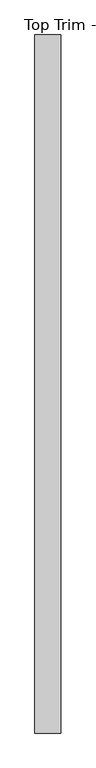
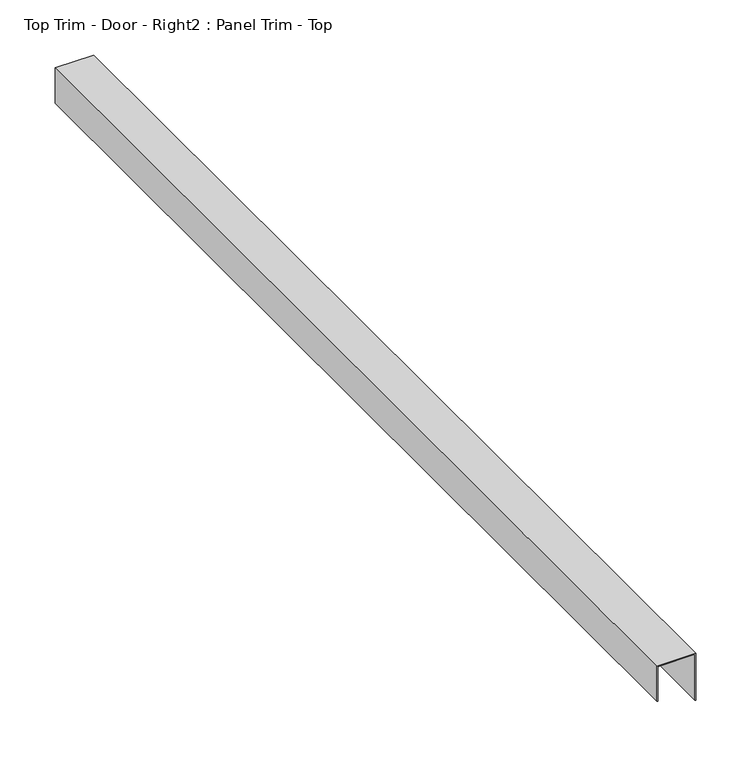
"""IFC4 building model written with IfcOpenShell, lengths in millimetres: proxy geometry, Top Trim - Door - Right2 : Panel Trim - Top."""

from ifc_helpers import new_model, si_unit, frame, origin, place, context, project, spatial, polyline, outline, extrude, source, transform, mapped, element, save


def top_trim_door_right2_panel_trim_top_ba49df41(model_context):
    return source(origin(), model_context, "Body", "SweptSolid", [
        extrude(outline(polyline([(2438.4, 587327.0060739), (2438.4, 587365.8934739), (2387.6, 587365.8934739), (2387.6, 587366.6808739), (2439.19375, 587366.6808739), (2439.19375, 587326.2186739), (2400.3, 587326.2186739), (2400.3, 587327.0060739), (2438.4, 587327.0060739)])), frame((0.0, -533976.0163841, 0.0), z_axis=(0.0, 1.0, 0.0), x_axis=(0.0, 0.0, 1.0)), (0.0, 0.0, 1.0), 1092.2),
    ])


if __name__ == "__main__":
    model = new_model("IFC4")
    model_context = context("Model", 3, world=origin())
    ifc_project = project(units=[si_unit("LENGTHUNIT", "METRE", prefix="MILLI")], contexts=[model_context])
    site = spatial("IfcSite", under=ifc_project)
    building = spatial("IfcBuilding", under=site)
    placement = place(None, origin())
    top_trim_door_right2_panel_trim_top_shape = top_trim_door_right2_panel_trim_top_ba49df41(model_context)
    element("IfcBuildingElementProxy", 1, Name="Top Trim - Door - Right2 : Panel Trim - Top", ObjectType="Top Trim - Door - Right2 : Panel Trim - Top", at=placement, inside=building, context=model_context, shape_type="MappedRepresentation", body=[
        mapped(top_trim_door_right2_panel_trim_top_shape, transform((0.0, 0.0, 0.0), x_axis=(1.0, 0.0, 0.0), y_axis=(0.0, 1.0, 0.0), z_axis=(0.0, 0.0, 1.0))),
    ])
    save(model, "model.ifc")

# Revit data of these elements
# Element 1 (IfcBuildingElementProxy, "Top Trim - Door - Right2 : Panel Trim - Top")
#   Materials on its faces: "EDGE TRIM BY MTL PANEL MFR."
# Materials
#   "EDGE TRIM BY MTL PANEL MFR.": class "Generic", colour RGB 239 242 240, transparency 0, Cost = 0
